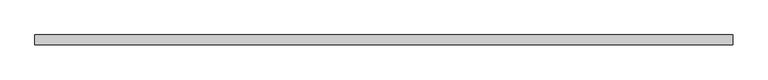
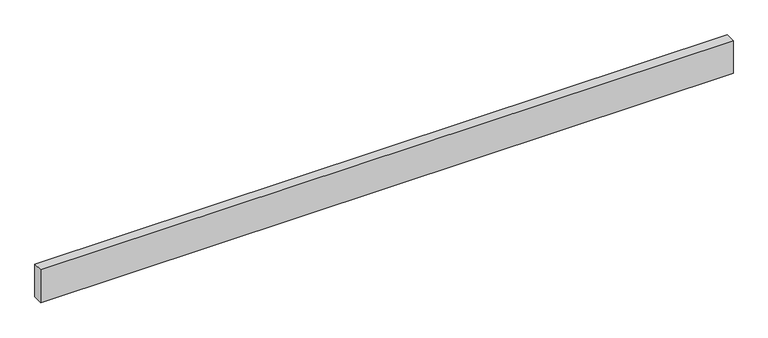
"""IFC4 building model written with IfcOpenShell, lengths in millimetres: beam geometry, NLRS_28_SF_LIB_houten balk-MMBW-SRP_gen_rsf : houten balk_gen__bxh 70x195."""

from ifc_helpers import new_model, si_unit, frame, origin, place, context, project, spatial, polyline, outline, extrude, source, transform, mapped, element, save


def beam_80e5a63c(model_context):
    return source(origin(), model_context, "Body", "SweptSolid", [
        extrude(outline(polyline([(-2451.0, -35.0), (-2451.0, 35.0), (2451.0, 35.0), (2451.0, -35.0), (-2451.0, -35.0)])), frame((0.0, 0.0, -122.5), z_axis=(0.0, 0.0, 1.0), x_axis=(1.0, 0.0, 0.0)), (0.0, 0.0, 1.0), 245.0),
    ])


if __name__ == "__main__":
    model = new_model("IFC4")
    model_context = context("Model", 3, world=origin())
    ifc_project = project(units=[si_unit("LENGTHUNIT", "METRE", prefix="MILLI")], contexts=[model_context])
    site = spatial("IfcSite", under=ifc_project)
    building = spatial("IfcBuilding", under=site)
    placement = place(None, origin())
    beam_shape = beam_80e5a63c(model_context)
    element("IfcBeam", 1, ObjectType="NLRS_28_SF_LIB_houten balk-MMBW-SRP_gen_rsf : houten balk_gen__bxh 70x195", at=placement, inside=building, context=model_context, shape_type="MappedRepresentation", body=[
        mapped(beam_shape, transform((0.0, 0.0, 0.0), x_axis=(1.0, 0.0, 0.0), y_axis=(0.0, 1.0, 0.0), z_axis=(0.0, 0.0, 1.0))),
    ])
    save(model, "model.ifc")

# Revit data of these elements
# Type "NLRS_28_SF_LIB_houten balk-MMBW-SRP_gen_rsf : houten balk_gen__bxh 70x195"
#   Type IfcGUID = "07M7mRoiH1CR8m_RSKIvYS"
#   IfcExportAs = "IfcBeamType"
#   Type Comments = "70x195"
#   Model = " "
#   Manufacturer = " "
#   Fire Rating = " "
#   Description = "houten balk 70x195"
#   Assembly Code = "28.11"
#   NLRS_C_lengte [instance default] = 3000 mm
#   NLRS_C_hoogte = 245 mm
#   NLRS_C_breedte = 70 mm
#   Length [instance default] = 3000 mm
#   Structural Material = NLRS_i2_hout naaldhout vuren_gen_rsf
#   Keynote = ""
# Element 1 (IfcBeam, "NLRS_28_SF_LIB_houten balk-MMBW-SRP_gen_rsf : houten balk_gen__bxh 70x195")
#   NLRS_C_lengte = 4972 mm
#   Materials on its faces: "NLRS_i2_hout naaldhout vuren_gen_rsf"
# Materials
#   "NLRS_i2_hout naaldhout vuren_gen_rsf": class "I - Hout", colour RGB 234 199 147, transparency 0, Keynote = "i2", Manufacturer = "Revit Standards Foundation", URL = "www.revitstandards.org", Description = "hout vuren", Cost = 0
